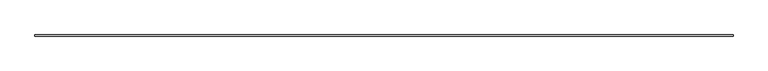
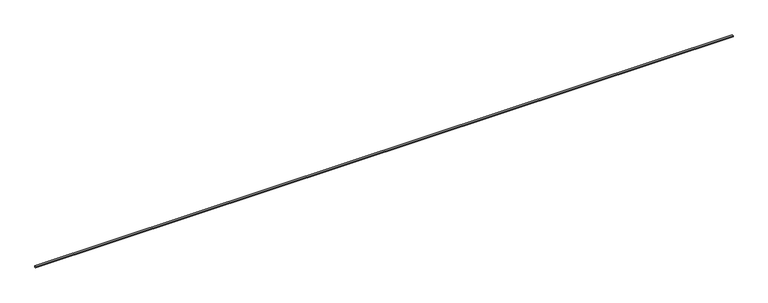
"""IFC4 building model written with IfcOpenShell, lengths in millimetres: proxy geometry, Joint004 2239 : Joint004 2239."""

import ifcopenshell
import ifcopenshell.guid

model = None  # the IFC model being written
_history = None  # IfcOwnerHistory: only IFC2X3 demands one
_inside = {}  # id of a spatial element -> (the spatial element, [elements in it])
_under = {}  # id of a project, library or spatial element -> (it, [spatial elements below it])
_declared = {}  # id of a project -> (the project, [libraries it declares])
_typed = {}  # id of a type object -> (the type object, [elements of that type])
_made_of = {}  # id of a material, layer set ... -> (it, [elements and type objects made of it])


def new_model(schema):
    """Start an empty IFC model of exactly this schema.

    Asked for "IFC4X3", IfcOpenShell would pick the latest addendum, in which some entities
    have other attributes; the version numbers below select the first issue.
    IFC2X3 requires an IfcOwnerHistory on every rooted entity: one is made here for all.
    """
    global model, _history
    if schema == "IFC4X3":
        model = ifcopenshell.file(schema_version=(4, 3, 0, 0))
    else:
        model = ifcopenshell.file(schema=schema)
    _inside.clear()
    _under.clear()
    _declared.clear()
    _typed.clear()
    _made_of.clear()
    _history = None
    if model.schema == "IFC2X3":
        org = make("IfcOrganization", Name="unknown")
        user = make(
            "IfcPersonAndOrganization",
            ThePerson=make("IfcPerson", FamilyName="unknown"),
            TheOrganization=org,
        )
        app = make(
            "IfcApplication",
            ApplicationDeveloper=org,
            Version="unknown",
            ApplicationFullName="unknown",
            ApplicationIdentifier="unknown",
        )
        _history = make(
            "IfcOwnerHistory",
            OwningUser=user,
            OwningApplication=app,
            ChangeAction="ADDED",
            CreationDate=0,
        )
    return model


def make(cls, **values):
    """One entity of the class cls with the attributes given. An attribute that is None is left unset."""
    return model.create_entity(
        cls, **{name: value for name, value in values.items() if value is not None}
    )


def rooted(cls, **values):
    """An entity with a GlobalId (a new one), such as an element, a storey or a relation."""
    return make(cls, GlobalId=ifcopenshell.guid.new(), OwnerHistory=_history, **values)


def si_unit(unit_type, name, prefix=None):
    """IfcSIUnit, for example si_unit("LENGTHUNIT", "METRE", prefix="MILLI")."""
    return make("IfcSIUnit", UnitType=unit_type, Prefix=prefix, Name=name)


def assignment(units):
    """IfcUnitAssignment: the units of a project."""
    return None if units is None else make("IfcUnitAssignment", Units=units)


def point(xyz):
    """IfcCartesianPoint."""
    return None if xyz is None else make("IfcCartesianPoint", Coordinates=xyz)


def direction(xyz):
    """IfcDirection."""
    return None if xyz is None else make("IfcDirection", DirectionRatios=xyz)


def frame(location, z_axis=None, x_axis=None):
    """IfcAxis2Placement3D, a coordinate frame: its origin and axes. An axis left out is left unset."""
    return make(
        "IfcAxis2Placement3D",
        Location=point(location),
        Axis=direction(z_axis),
        RefDirection=direction(x_axis),
    )


def frame_2d(location, x_axis=None):
    """IfcAxis2Placement2D, a coordinate frame in the plane: its origin and x axis."""
    return make(
        "IfcAxis2Placement2D", Location=point(location), RefDirection=direction(x_axis)
    )


def origin():
    """The frame at (0, 0, 0) with its axes left unset."""
    return frame((0.0, 0.0, 0.0))


def place(relative_to, where):
    """IfcLocalPlacement: puts the frame where relative to a parent placement (None: the world)."""
    return make(
        "IfcLocalPlacement", PlacementRelTo=relative_to, RelativePlacement=where
    )


def context(
    kind, dimensions, precision=None, world=None, true_north=None, identifier=None
):
    """IfcGeometricRepresentationContext, for example the 3D "Model" context."""
    return make(
        "IfcGeometricRepresentationContext",
        ContextIdentifier=identifier,
        ContextType=kind,
        CoordinateSpaceDimension=dimensions,
        Precision=precision,
        WorldCoordinateSystem=world,
        TrueNorth=true_north,
    )


def project(units=None, contexts=None):
    """IfcProject with its units and contexts."""
    return rooted(
        "IfcProject",
        Name="project",
        RepresentationContexts=contexts,
        UnitsInContext=assignment(units),
    )


def spatial(cls, under=None, at=None, **own):
    """A site, building, storey or space (cls), placed at a placement, below another one or the project."""
    s = rooted(cls, ObjectPlacement=at, **own)
    if under is not None:
        _under.setdefault(under.id(), (under, []))[1].append(s)
    return s


def polyline(points):
    """IfcPolyline through the points."""
    return make("IfcPolyline", Points=[point(p) for p in points])


def circle_curve(where, radius):
    """IfcCircle in the frame where."""
    return make("IfcCircle", Position=where, Radius=radius)


def trimmed(basis, trim1, trim2, sense, master):
    """IfcTrimmedCurve: the piece of a basis curve between two trims."""
    return make(
        "IfcTrimmedCurve",
        BasisCurve=basis,
        Trim1=trim1,
        Trim2=trim2,
        SenseAgreement=sense,
        MasterRepresentation=master,
    )


def segment(curve, same_sense, transition):
    """IfcCompositeCurveSegment."""
    return make(
        "IfcCompositeCurveSegment",
        Transition=transition,
        SameSense=same_sense,
        ParentCurve=curve,
    )


def composite_curve(segments, self_intersect=None):
    """IfcCompositeCurve: segments joined end to end."""
    return make("IfcCompositeCurve", Segments=segments, SelfIntersect=self_intersect)


def outline(outer, holes=None, kind="AREA"):
    """IfcArbitraryClosedProfileDef: a profile drawn as a closed curve; with holes, ...WithVoids."""
    if holes is None:
        return make("IfcArbitraryClosedProfileDef", ProfileType=kind, OuterCurve=outer)
    return make(
        "IfcArbitraryProfileDefWithVoids",
        ProfileType=kind,
        OuterCurve=outer,
        InnerCurves=holes,
    )


def extrude(swept, where, along, depth):
    """IfcExtrudedAreaSolid: the profile swept, set in the frame where, extruded along a direction by depth."""
    return make(
        "IfcExtrudedAreaSolid",
        SweptArea=swept,
        Position=where,
        ExtrudedDirection=direction(along),
        Depth=depth,
    )


def shape(context_of_items, identifier, shape_type, items):
    """IfcShapeRepresentation: the items that make up one representation, for example the "Body"."""
    return make(
        "IfcShapeRepresentation",
        ContextOfItems=context_of_items,
        RepresentationIdentifier=identifier,
        RepresentationType=shape_type,
        Items=items,
    )


def source(mapping_origin, context_of_items, identifier, shape_type, items):
    """IfcRepresentationMap: a shape defined once, which mapped items show again and again."""
    return make(
        "IfcRepresentationMap",
        MappingOrigin=mapping_origin,
        MappedRepresentation=shape(context_of_items, identifier, shape_type, items),
    )


def transform(
    local_origin,
    x_axis=None,
    y_axis=None,
    z_axis=None,
    scale=None,
    scale2=None,
    scale3=None,
    uniform=True,
):
    """IfcCartesianTransformationOperator3D, or its non-uniform kind. x_axis, y_axis, z_axis: its Axis1, 2, 3."""
    if uniform:
        return make(
            "IfcCartesianTransformationOperator3D",
            Axis1=direction(x_axis),
            Axis2=direction(y_axis),
            LocalOrigin=point(local_origin),
            Scale=scale,
            Axis3=direction(z_axis),
        )
    return make(
        "IfcCartesianTransformationOperator3DnonUniform",
        Axis1=direction(x_axis),
        Axis2=direction(y_axis),
        LocalOrigin=point(local_origin),
        Scale=scale,
        Axis3=direction(z_axis),
        Scale2=scale2,
        Scale3=scale3,
    )


def mapped(mapping_source, mapping_target):
    """IfcMappedItem: shows the shape of a source again, moved by a transform."""
    return make(
        "IfcMappedItem", MappingSource=mapping_source, MappingTarget=mapping_target
    )


def made_of(thing, what):
    """Note that an element or type object is made of a material, layer set ...; save() writes the relation."""
    if what is not None:
        _made_of.setdefault(what.id(), (what, []))[1].append(thing)
    return thing


def element(
    cls,
    number,
    at=None,
    inside=None,
    cuts=None,
    type_object=None,
    material=None,
    context=None,
    identifier="Body",
    shape_type=None,
    held_by="IfcProductDefinitionShape",
    body=None,
    shapes=None,
    **own,
):
    """One element of the class cls, such as IfcWall. Its Tag is "e" and its number.

    at: its placement. inside: the storey or other place that contains it. cuts: it is an
    opening in that element (IfcRelVoidsElement). A single representation is given by context,
    identifier, shape_type and body (its items); several are given by shapes. held_by: the class
    of the entity that holds the representations. save() writes the other relations.
    """
    e = rooted(cls, Tag="e%d" % number, ObjectPlacement=at, **own)
    if body is not None:
        shapes = [shape(context, identifier, shape_type, body)]
    if shapes is not None:
        e.Representation = make(held_by, Representations=shapes)
    if inside is not None:
        _inside.setdefault(inside.id(), (inside, []))[1].append(e)
    if cuts is not None:
        rooted(
            "IfcRelVoidsElement", RelatingBuildingElement=cuts, RelatedOpeningElement=e
        )
    if type_object is not None:
        _typed.setdefault(type_object.id(), (type_object, []))[1].append(e)
    return made_of(e, material)


def aggregate(whole, parts):
    """IfcRelAggregates: a whole, such as a stair, and the parts it consists of."""
    return rooted("IfcRelAggregates", RelatingObject=whole, RelatedObjects=parts)


def save(model, path):
    """Write the relations noted so far, then the file.

    IfcRelAggregates (storeys below a building ...), IfcRelContainedInSpatialStructure (elements
    in a storey), IfcRelDefinesByType, IfcRelAssociatesMaterial and IfcRelDeclares: one each for
    every whole, place, type object, material and project.
    """
    for whole, parts in _under.values():
        aggregate(whole, parts)
    for where, things in _inside.values():
        rooted(
            "IfcRelContainedInSpatialStructure",
            RelatedElements=things,
            RelatingStructure=where,
        )
    for kind, things in _typed.values():
        rooted("IfcRelDefinesByType", RelatedObjects=things, RelatingType=kind)
    for what, things in _made_of.values():
        rooted("IfcRelAssociatesMaterial", RelatedObjects=things, RelatingMaterial=what)
    for by, libraries in _declared.values():
        rooted("IfcRelDeclares", RelatingContext=by, RelatedDefinitions=libraries)
    model.write(path)


def generic_models_4fac969d(model_context):
    return source(origin(), model_context, "Body", "SweptSolid", [
        extrude(outline(composite_curve([segment(polyline([(10405.3793386, 40791.3953125), (10405.3793386, 40795.3132812)]), True, "CONTINUOUS"), segment(trimmed(circle_curve(frame_2d((10406.9776706, 40800.4851562)), 5.4132205), [point((10405.3793386, 40795.3132812))], [point((10408.5760026, 40795.3132812))], True, "CARTESIAN"), True, "CONTINUOUS"), segment(polyline([(10408.5760026, 40795.3132812), (10408.5760026, 40791.3953125)]), True, "CONTINUOUS"), segment(trimmed(circle_curve(frame_2d((10406.9776706, 40796.5671875)), 5.4132205), [point((10408.5760026, 40791.3953125))], [point((10405.3793386, 40791.3953125))], False, "CARTESIAN"), True, "CONTINUOUS")], self_intersect=False)), frame((3694.2883192, 0.0, 0.0), z_axis=(1.0, 0.0, 0.0), x_axis=(0.0, 1.0, 0.0)), (0.0, 0.0, 1.0), 2000.0),
    ])


if __name__ == "__main__":
    model = new_model("IFC4")
    model_context = context("Model", 3, world=origin())
    ifc_project = project(units=[si_unit("LENGTHUNIT", "METRE", prefix="MILLI")], contexts=[model_context])
    site = spatial("IfcSite", under=ifc_project)
    building = spatial("IfcBuilding", under=site)
    placement = place(None, origin())
    generic_models_shape = generic_models_4fac969d(model_context)
    element("IfcBuildingElementProxy", 1, Name="Joint004 2239 : Joint004 2239", ObjectType="Joint004 2239 : Joint004 2239", at=placement, inside=building, context=model_context, shape_type="MappedRepresentation", body=[
        mapped(generic_models_shape, transform((0.0, 0.0, 0.0), x_axis=(1.0, 0.0, 0.0), y_axis=(0.0, 1.0, 0.0), z_axis=(0.0, 0.0, 1.0))),
    ])
    save(model, "model.ifc")

# Revit data of these elements
# Type "Joint004 2239 : Joint004 2239"
#   NameOverride = "Joint004"
# Element 1 (IfcBuildingElementProxy, "Joint004 2239 : Joint004 2239")
#   Materials on its faces: "SILICON JOINT"
# Materials
#   "SILICON JOINT": class "Unassigned", colour RGB 150 184 127, transparency 0
